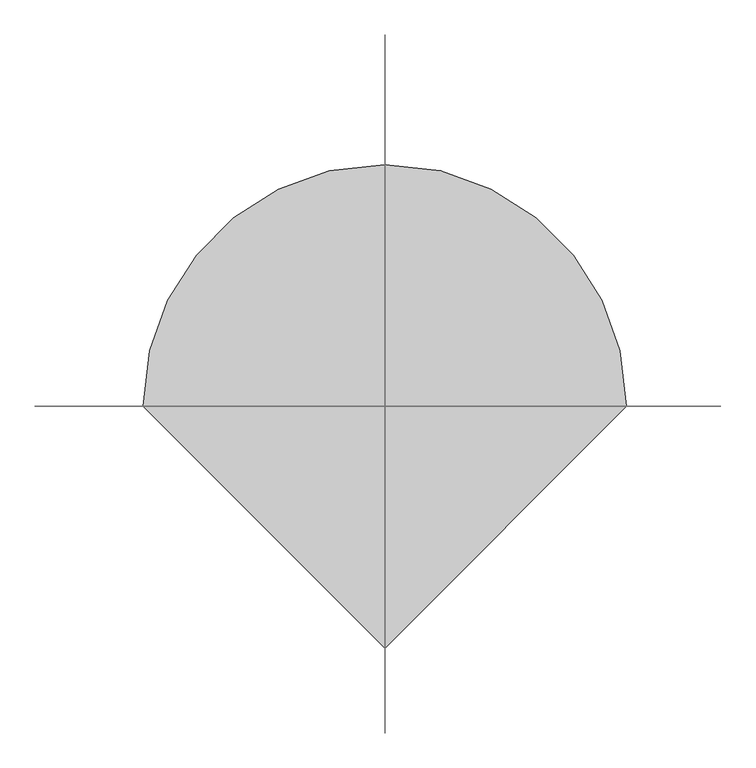
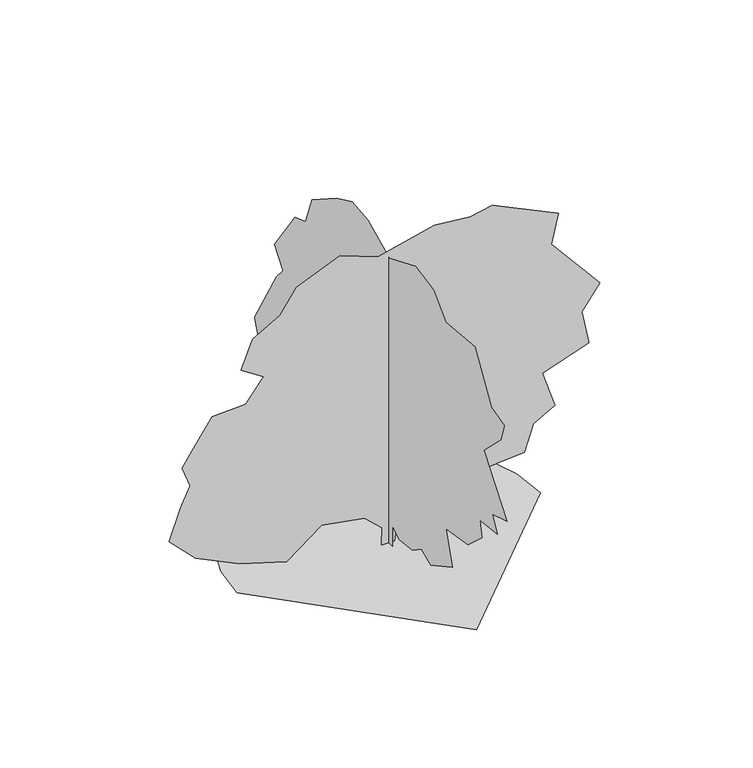
"""IFC4 building model written with IfcOpenShell, lengths in millimetres: proxy geometry, hibiscus syriacus 26076 : hibiscus syriacus 26076."""

from ifc_helpers import new_model, si_unit, origin, place, context, project, spatial, triangles, source, transform, mapped, element, save


def entourage_ec5c78c5(model_context):
    return source(origin(), model_context, "Body", "Tessellation", [
        triangles([(-718.2296339, 0.0, 5.8e-05), (-699.2430748, 164.5709867, 5.8e-05), (-645.166361, 315.7023142, 5.8e-05), (-560.3301876, 449.0652858, 5.8e-05), (-449.0652858, 560.3301876, 5.8e-05), (-315.7023142, 645.166361, 5.8e-05), (-164.5707324, 699.2430748, 5.8e-05), (3.14e-05, 718.2296339, 5.8e-05), (164.5709867, 699.2430748, 5.8e-05), (315.7023142, 645.166361, 5.8e-05), (449.0652858, 560.3301876, 5.8e-05), (560.3301876, 449.0652858, 5.8e-05), (645.166361, 315.7023142, 5.8e-05), (699.2430748, 164.5707324, 5.8e-05), (718.2296339, -6.28e-05, 5.8e-05), (-9.42e-05, -718.2296339, 5.8e-05), (-34.4417068, -8.54e-05, 0.0004029), (-31.4201161, -7.54e-05, 85.3357887), (-116.0190539, -6.6e-05, 163.8917949), (-318.4505839, -6.17e-05, 200.1483391), (-484.6279043, -7.68e-05, 73.2501891), (-708.2093153, -6.85e-05, 142.7419322), (-916.6853256, -5.67e-05, 242.4475559), (-1040.5638834, -4.15e-05, 369.3446795), (-986.1773048, -2.35e-05, 520.4140194), (-940.856016, -1.24e-05, 614.076689), (-980.1346504, -1e-07, 716.8046482), (-931.7932697, 8.2e-06, 786.2967001), (-838.1305275, 2.47e-05, 925.2806585), (-677.9959705, 2.55e-05, 931.323313), (-593.398518, 3.84e-05, 1040.0939993), (-699.1465691, 4.67e-05, 1109.5859785), (-644.762534, 6.29e-05, 1245.5473743), (-514.8412491, 7.16e-05, 1318.0593727), (-436.2865236, 8.53e-05, 1432.8727135), (-230.8316043, 9.53e-05, 1517.4726368), (-52.5699789, 8.74e-05, 1451.0008221), (216.3332524, 9.5e-05, 1514.4501469), (385.5321362, 9.28e-05, 1496.3220383), (491.2801509, 9.53e-05, 1517.4726368), (802.4816133, 7.77e-05, 1369.4233887), (769.2456333, 6.04e-05, 1224.3967758), (998.8722422, 2.8e-05, 952.4739841), (914.2723188, 1.43e-05, 837.6606434), (947.5082262, -5.9e-06, 668.4632675), (726.946907, -1.49e-05, 592.9286339), (787.37614, -3.65e-05, 411.6459128), (684.6481808, -4.3e-05, 357.2593343), (642.3495272, -5.85e-05, 227.340611), (237.483106, -6.21e-05, 197.1267394), (140.7988277, -7.07e-05, 124.6136692), (53.1785627, -6.42e-05, 178.9984673), (25.9860297, -8.59e-05, 0.0), (-0.0007807, -31.0927106, 0.000457), (-0.0007807, -31.0927106, 100.9481805), (-0.0007869, -87.072138, 68.5389896), (-0.0007995, -193.1381747, 80.3241033), (-0.0008058, -269.7409118, 130.4109715), (-0.0008121, -346.3449205, 98.0017761), (-0.0008373, -520.1752622, 192.282958), (-0.0008373, -470.0888935, 354.3281542), (-0.0008562, -649.8120077, 383.7922351), (-0.0008688, -764.7167673, 489.857745), (-0.0008688, -747.0383406, 566.4617901), (-0.0008877, -891.4071447, 584.1376734), (-0.0008814, -850.1600258, 657.7952414), (-0.0009003, -970.9575943, 696.098572), (-0.0008877, -782.3951941, 937.693709), (-0.0009066, -920.8711893, 1073.2207563), (-0.0009066, -950.3327631, 1161.6103466), (-0.0009003, -841.3208124, 1188.1254433), (-0.000894, -705.7912216, 1409.0982925), (-0.0008688, -470.0888935, 1388.4733887), (-0.0008562, -366.9697881, 1488.6486694), (-0.0008436, -219.6545613, 1518.1102432), (-0.0008184, -4.575997, 1426.7767193), (-0.0007995, 172.2011714, 1509.2709572), (-0.0007869, 301.8364273, 1524.0030521), (-0.0007744, 431.473191, 1462.131102), (-0.0007492, 628.8747683, 1335.4407246), (-0.0007366, 684.8539822, 1191.0718477), (-0.0007303, 770.297168, 1161.6103466), (-0.0007051, 938.2346643, 925.9080185), (-0.0007114, 867.5235008, 834.5720238), (-0.0007051, 920.5562376, 772.700001), (-0.0006736, 1103.2258289, 460.3937004), (-0.0006736, 1020.7315184, 251.2085401), (-0.0006988, 811.5442869, 209.9606217), (-0.0007555, 275.3213124, 192.282958), (-0.0007744, 60.2420624, 183.443999), (-0.0007744, 30.7792736, 0.0004496)], [[16, 15, 1], [15, 14, 1], [1, 14, 2], [14, 13, 2], [2, 13, 3], [3, 13, 4], [13, 12, 4], [12, 11, 4], [4, 11, 5], [5, 11, 6], [6, 11, 7], [7, 11, 8], [8, 11, 9], [9, 11, 10], [17, 53, 18], [53, 52, 18], [18, 52, 19], [45, 44, 46], [47, 46, 48], [32, 31, 33], [41, 40, 42], [43, 42, 44], [33, 31, 34], [51, 50, 52], [49, 48, 50], [24, 23, 25], [48, 46, 50], [44, 42, 46], [40, 39, 42], [42, 39, 46], [46, 39, 50], [39, 38, 50], [38, 37, 50], [50, 37, 52], [52, 37, 19], [19, 37, 20], [37, 36, 20], [36, 35, 20], [35, 34, 20], [34, 31, 20], [31, 30, 20], [20, 30, 21], [21, 30, 22], [22, 30, 23], [23, 30, 25], [25, 30, 26], [30, 29, 26], [29, 28, 26], [26, 28, 27], [65, 64, 66], [67, 66, 68], [70, 69, 71], [54, 91, 55], [91, 90, 55], [69, 68, 71], [60, 59, 61], [59, 58, 61], [83, 82, 84], [72, 71, 73], [71, 68, 73], [66, 64, 68], [63, 62, 64], [87, 86, 88], [86, 85, 88], [88, 85, 89], [85, 84, 89], [84, 82, 89], [82, 81, 89], [89, 81, 90], [81, 80, 90], [80, 79, 90], [79, 78, 90], [78, 77, 90], [77, 76, 90], [76, 75, 90], [75, 74, 90], [74, 73, 90], [73, 68, 90], [68, 64, 90], [90, 64, 55], [55, 64, 56], [62, 61, 64], [64, 61, 56], [61, 58, 56], [56, 58, 57]], closed=False),
    ])


if __name__ == "__main__":
    model = new_model("IFC4")
    model_context = context("Model", 3, world=origin())
    ifc_project = project(units=[si_unit("LENGTHUNIT", "METRE", prefix="MILLI")], contexts=[model_context])
    site = spatial("IfcSite", under=ifc_project)
    building = spatial("IfcBuilding", under=site)
    placement = place(None, origin())
    entourage_shape = entourage_ec5c78c5(model_context)
    element("IfcBuildingElementProxy", 1, Name="hibiscus syriacus 26076 : hibiscus syriacus 26076", ObjectType="hibiscus syriacus 26076 : hibiscus syriacus 26076", at=placement, inside=building, context=model_context, shape_type="MappedRepresentation", body=[
        mapped(entourage_shape, transform((0.0, 0.0, 0.0), x_axis=(1.0, 0.0, 0.0), y_axis=(0.0, 1.0, 0.0), z_axis=(0.0, 0.0, 1.0))),
    ])
    save(model, "model.ifc")

# Revit data of these elements
# Type "hibiscus syriacus 26076 : hibiscus syriacus 26076"
#   built-in parameter 1005195 = "RPC-16-FVPE-AH00-2TUK-G000-ST1L-LVER-AU"
#   Height = 0
